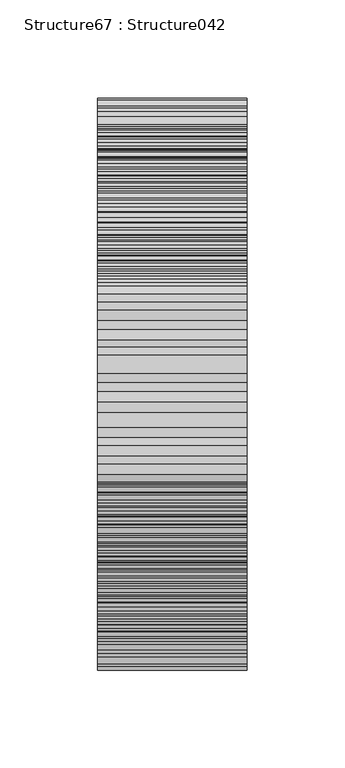
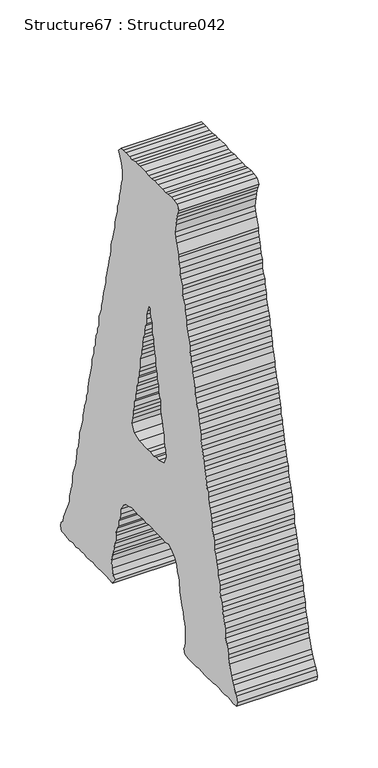
"""IFC4 building model written with IfcOpenShell, lengths in millimetres: proxy geometry, Structure67 : Structure042."""

from ifc_helpers import new_model, si_unit, frame, origin, place, context, project, spatial, polyline, outline, extrude, source, transform, mapped, element, save


def structure67_structure042_b80fde91(model_context):
    return source(origin(), model_context, "Body", "SweptSolid", [
        extrude(outline(polyline([(276286.8104308, 3818.8310229), (276286.8104308, 3814.7296538), (276287.9914198, 3811.2043377), (276290.3084687, 3805.9476534), (276290.3084687, 3801.8462843), (276290.9101953, 3795.960595), (276293.2497087, 3791.8865042), (276293.2497087, 3787.7867397), (276295.6132911, 3783.0868532), (276296.1925533, 3777.8285642), (276296.1925533, 3773.11905), (276298.5320667, 3769.6274306), (276298.5320667, 3763.759392), (276300.2923178, 3759.6596275), (276302.0541736, 3755.559863), (276302.0541736, 3750.8583719), (276303.212698, 3746.1745313), (276305.5522114, 3737.400554), (276306.7332003, 3732.1149867), (276307.8917247, 3727.4311462), (276309.0743182, 3723.3313817), (276309.0743182, 3718.6571688), (276310.8345694, 3713.3555556), (276311.436296, 3709.2718371), (276313.1740827, 3704.5879966), (276314.3326072, 3701.0723082), (276314.9343338, 3695.786741), (276316.6961896, 3690.512406), (276316.6961896, 3685.8285655), (276317.8771785, 3682.8857208), (276319.0357029, 3677.6274319), (276320.7959541, 3672.9435914), (276322.5562052, 3668.8261762), (276323.1354674, 3664.1423357), (276323.7163343, 3660.0682449), (276324.3180609, 3654.1841602), (276326.6575743, 3650.1004418), (276327.259301, 3645.9830266), (276327.8160987, 3641.2991861), (276328.395361, 3636.0408972), (276329.5763499, 3631.915459), (276331.3382056, 3627.8397636), (276333.0984567, 3622.555801), (276334.2794456, 3617.2718384), (276334.2794456, 3613.772196), (276334.8587079, 3607.8961343), (276336.618959, 3604.3964919), (276337.7774834, 3600.2967274), (276338.960077, 3595.5872132), (276339.5393392, 3589.7544759), (276340.7203281, 3586.2115092), (276344.8200926, 3577.4535778), (276347.1612105, 3572.1423369), (276348.9214617, 3568.6426945), (276350.0799861, 3563.366755), (276353.0212262, 3560.441561), (276354.2038197, 3556.3417965), (276352.4194995, 3551.6675836), (276347.7629372, 3551.6675836), (276343.0598414, 3551.0658569), (276338.960077, 3550.4833855), (276333.7001834, 3551.6675836), (276328.395361, 3550.4833855), (276323.7163343, 3551.6675836), (276320.1942274, 3551.0658569), (276314.3326072, 3551.6675836), (276310.8345694, 3551.0658569), (276304.9954136, 3551.0658569), (276300.87158, 3551.6675836), (276296.7718156, 3551.0658569), (276292.0687198, 3551.0658569), (276287.3896931, 3551.6675836), (276278.0284304, 3551.6675836), (276273.3494037, 3551.0658569), (276268.0445813, 3550.4833855), (276264.5465435, 3556.3417965), (276267.465319, 3559.2669905), (276269.2255702, 3565.1254015), (276269.8048324, 3572.7440636), (276268.0445813, 3578.6104977), (276266.3067946, 3582.7102621), (276265.7275324, 3587.3860796), (276265.1258057, 3592.0955938), (276262.7846877, 3596.7698067), (276262.7846877, 3601.4536473), (276262.2054255, 3604.9709403), (276261.0244366, 3610.2292293), (276258.6849232, 3613.772196), (276258.105661, 3619.6145609), (276256.3438053, 3622.555801), (276255.1628164, 3627.8397636), (276255.1628164, 3633.0980525), (276250.4837897, 3639.5405396), (276246.9616828, 3643.0578326), (276239.9415381, 3644.8245022), (276236.4210359, 3645.9830266), (276230.5594156, 3645.4262289), (276226.4580466, 3644.8245022), (276221.7790198, 3645.4262289), (276217.0759241, 3645.9830266), (276212.998624, 3644.8245022), (276207.6938016, 3645.4262289), (276195.4137634, 3645.4262289), (276189.5521432, 3644.8245022), (276180.1700207, 3644.8245022), (276175.490994, 3645.9830266), (276169.0501115, 3642.4833842), (276164.926278, 3638.9580681), (276162.0299668, 3633.0980525), (276160.8489779, 3627.2396415), (276159.0871222, 3622.555801), (276157.9061333, 3619.6145609), (276156.7251444, 3609.0723094), (276155.5441555, 3604.3964919), (276154.4080955, 3600.2967274), (276152.6462398, 3596.1953583), (276151.4652508, 3592.0955938), (276150.8859886, 3586.2115092), (276149.103273, 3582.7102621), (276147.9447486, 3578.6104977), (276147.9447486, 3573.9266571), (276147.9447486, 3563.9412034), (276149.103273, 3559.2669905), (276150.8859886, 3555.7416744), (276148.5240108, 3551.6675836), (276143.2641173, 3550.4833855), (276129.7806257, 3550.4833855), (276125.6808612, 3551.6675836), (276120.3985032, 3551.0658569), (276115.7194765, 3550.4833855), (276111.6181074, 3550.4833855), (276105.7564872, 3551.0658569), (276101.6791872, 3551.0658569), (276096.9760914, 3551.6675836), (276092.8747223, 3551.6675836), (276088.1732311, 3550.4833855), (276082.9133376, 3550.4833855), (276078.2327063, 3551.6675836), (276072.9294884, 3551.0658569), (276069.429846, 3550.4833855), (276063.5906902, 3551.0658569), (276062.4097013, 3555.1848766), (276064.1715571, 3560.441561), (276065.3300815, 3563.366755), (276068.8505838, 3568.6426945), (276070.6108349, 3572.1423369), (276072.3726907, 3576.2693797), (276075.2914662, 3586.2115092), (276077.0517174, 3590.3289243), (276077.0517174, 3594.4286888), (276078.2327063, 3599.1125293), (276079.3928353, 3604.3964919), (276081.7323487, 3608.4705827), (276082.3116109, 3612.5976255), (276082.3116109, 3617.2718384), (276083.4925998, 3622.555801), (276085.2528509, 3627.2396415), (276085.8545776, 3632.5155811), (276087.0147067, 3636.0408972), (276088.1732311, 3640.114988), (276089.9334823, 3645.4262289), (276091.1144712, 3650.6845178), (276091.1144712, 3655.3587307), (276092.2954601, 3659.4584952), (276094.636578, 3663.5598643), (276094.636578, 3668.8261762), (276096.3743647, 3673.5276674), (276096.9760914, 3677.0449605), (276098.7363425, 3682.8857208), (276099.894867, 3686.4030139), (276099.894867, 3691.0868544), (276100.4965936, 3695.2122926), (276101.6791872, 3699.8881101), (276103.9962361, 3705.7545441), (276103.9962361, 3710.4560353), (276105.177225, 3714.5301261), (276106.3357494, 3718.0554422), (276107.5167383, 3723.3313817), (276109.2785941, 3727.4311462), (276110.4371185, 3732.7167134), (276110.4371185, 3737.9750024), (276112.1973696, 3740.9162424), (276113.3783585, 3745.6000829), (276113.9576208, 3751.4424479), (276115.7194765, 3756.1423345), (276116.9004654, 3759.6596275), (276117.4572632, 3764.3611187), (276118.0589899, 3769.0176809), (276119.819241, 3774.3032481), (276120.3985032, 3777.8285642), (276122.1587543, 3783.0868532), (276122.1587543, 3788.3611881), (276123.3413479, 3791.8865042), (276125.0791345, 3797.1463977), (276125.6808612, 3801.8462843), (276126.8393857, 3806.5317294), (276127.4411123, 3810.0474179), (276129.7806257, 3815.3313805), (276130.9632192, 3820.015221), (276132.1442081, 3824.1149855), (276132.1442081, 3829.374879), (276135.0629837, 3837.6000817), (276136.2215081, 3842.8583706), (276136.8232348, 3846.9757858), (276138.5850906, 3851.6612309), (276138.5850906, 3856.9179152), (276140.3228772, 3861.0192843), (276140.9021395, 3866.3032469), (276141.5038661, 3869.8189354), (276143.2641173, 3873.9203044), (276145.0243684, 3878.5784713), (276146.2069619, 3883.8881076), (276146.2069619, 3888.5623205), (276147.3654864, 3892.6636896), (276149.103273, 3897.3475301), (276149.103273, 3902.6314927), (276151.4652508, 3906.1487857), (276152.6462398, 3910.8310217), (276153.2271066, 3916.0909152), (276153.2271066, 3919.6066036), (276155.5441555, 3924.2888396), (276156.7251444, 3928.9919353), (276157.3268711, 3934.2758979), (276158.4853955, 3938.9517154), (276159.6663844, 3944.235678), (276159.6663844, 3947.1496398), (276163.1660268, 3956.5349715), (276164.3470157, 3961.794865), (276165.5280046, 3965.8930249), (276163.7677535, 3974.7055128), (276162.5867646, 3979.9621971), (276162.0299668, 3983.4794902), (276160.8489779, 3987.5792547), (276158.4853955, 3991.6806238), (276162.0299668, 3996.390138), (276167.2882558, 3996.9645864), (276171.3671604, 3997.5486624), (276176.6719829, 3997.5486624), (276180.7492829, 3996.390138), (276186.0316409, 3996.9645864), (276193.6310478, 3996.9645864), (276198.9358702, 3997.5486624), (276204.1941592, 3996.390138), (276208.8747905, 3996.390138), (276213.5778863, 3997.5486624), (276222.9375443, 3997.5486624), (276227.0389134, 3996.9645864), (276230.5594156, 3997.5486624), (276235.8417736, 3996.390138), (276240.5208004, 3996.390138), (276245.7806939, 3997.5486624), (276249.9045274, 3997.5486624), (276253.9818275, 3996.9645864), (276258.105661, 3992.2614906), (276255.7645431, 3987.5792547), (276253.9818275, 3984.0635662), (276252.823303, 3979.3781211), (276251.6647786, 3974.7055128), (276251.6647786, 3966.5043792), (276253.4025652, 3962.3757319), (276254.5835542, 3957.1190475), (276255.1628164, 3952.435207), (276256.9246721, 3947.7337158), (276256.9246721, 3944.235678), (276258.105661, 3938.3499888), (276259.8659122, 3934.8503464), (276259.8659122, 3929.5904528), (276261.6036988, 3924.8905662), (276263.36395, 3919.6066036), (276264.5465435, 3915.5068392), (276264.5465435, 3910.8310217), (276265.7275324, 3906.1487857), (276266.9085213, 3902.6314927), (276268.0445813, 3896.763454), (276269.8048324, 3893.822214), (276270.9858213, 3888.5623205), (276270.9858213, 3884.4609514), (276271.587548, 3878.5784713), (276273.3494037, 3875.0772243), (276273.928666, 3870.4030114), (276275.0871904, 3866.3032469), (276276.2457149, 3861.0192843), (276277.4267038, 3856.9179152), (276279.1885595, 3851.6612309), (276279.1885595, 3846.9757858), (276280.9488106, 3841.6741725), (276281.5505373, 3838.1761347), (276283.288324, 3833.4730389), (276283.8675862, 3828.2163546), (276284.4693129, 3824.1149855), (276286.8104308, 3818.8310229)]), holes=[polyline([(276224.1185332, 3720.4158154), (276232.3196668, 3723.9154578), (276235.8417736, 3730.9323932), (276234.6607847, 3736.7988273), (276233.5006557, 3741.5003184), (276233.5006557, 3744.9999608), (276231.7179401, 3750.3015741), (276231.7179401, 3755.559863), (276229.9801534, 3759.0595054), (276229.4008912, 3764.3611187), (276228.2199023, 3768.4432325), (276228.2199023, 3773.11905), (276225.8787843, 3777.8285642), (276225.8787843, 3783.0868532), (276224.1185332, 3786.0280932), (276223.5168065, 3790.7039107), (276222.3807465, 3795.4037973), (276221.7790198, 3804.7730829), (276220.0187687, 3810.0474179), (276219.4379019, 3814.7296538), (276218.256913, 3818.8310229), (276217.6776508, 3822.932392), (276217.0759241, 3828.790803), (276214.7588752, 3833.4730389), (276214.7588752, 3836.9919366), (276214.1571485, 3842.2758992), (276211.8160305, 3845.8012153), (276211.8160305, 3851.0595042), (276211.2367683, 3855.7353217), (276209.4540527, 3860.4432313), (276208.2955283, 3865.1190488), (276206.5577416, 3864.5446004), (276206.5577416, 3860.4432313), (276205.3767527, 3856.3161885), (276203.614897, 3851.6612309), (276203.614897, 3846.3772683), (276203.0131703, 3842.2758992), (276200.6736569, 3837.6000817), (276200.6736569, 3832.8921721), (276200.0943947, 3828.790803), (276198.9358702, 3824.1149855), (276197.7548813, 3819.4150989), (276197.1740145, 3813.5743386), (276196.5722878, 3810.0474179), (276194.8120367, 3805.9476534), (276194.8120367, 3800.6717138), (276192.4725233, 3795.4037973), (276192.4725233, 3790.7039107), (276191.3139989, 3786.0280932), (276189.5521432, 3782.5027771), (276188.9728809, 3777.2444882), (276188.9728809, 3772.5606477), (276188.3711542, 3767.8607611), (276186.6109031, 3763.759392), (276186.0316409, 3759.6596275), (276185.4299142, 3754.9854146), (276183.1128653, 3750.8583719), (276183.6921275, 3744.9999608), (276182.5111386, 3740.9162424), (276181.3510096, 3736.7988273), (276180.1700207, 3730.9323932), (276183.1128653, 3723.3313817), (276191.8932611, 3720.4158154), (276195.9930256, 3720.9726131), (276200.0943947, 3719.8140887), (276205.3767527, 3720.9726131), (276210.6350416, 3720.4158154), (276224.1185332, 3720.4158154)])]), frame((-59031.6926606, 0.0, 0.0), z_axis=(1.0, 0.0, 0.0), x_axis=(0.0, 1.0, 0.0)), (0.0, 0.0, 1.0), 76.2),
    ])


if __name__ == "__main__":
    model = new_model("IFC4")
    model_context = context("Model", 3, world=origin())
    ifc_project = project(units=[si_unit("LENGTHUNIT", "METRE", prefix="MILLI")], contexts=[model_context])
    site = spatial("IfcSite", under=ifc_project)
    building = spatial("IfcBuilding", under=site)
    placement = place(None, origin())
    structure67_structure042_shape = structure67_structure042_b80fde91(model_context)
    element("IfcBuildingElementProxy", 1, Name="Structure67 : Structure042", ObjectType="Structure67 : Structure042", at=placement, inside=building, context=model_context, shape_type="MappedRepresentation", body=[
        mapped(structure67_structure042_shape, transform((0.0, 0.0, 0.0), x_axis=(1.0, 0.0, 0.0), y_axis=(0.0, 1.0, 0.0), z_axis=(0.0, 0.0, 1.0))),
    ])
    save(model, "model.ifc")

# Revit data of these elements
# Type "Structure67 : Structure042"
#   NameOverride = "Structure042"
# Element 1 (IfcBuildingElementProxy, "Structure67 : Structure042")
#   Materials on its faces: "BRUSHED ALUM. LETTERING"
# Materials
#   "BRUSHED ALUM. LETTERING": class "Unassigned", colour RGB 169 181 186, transparency 0, Cost = 0
